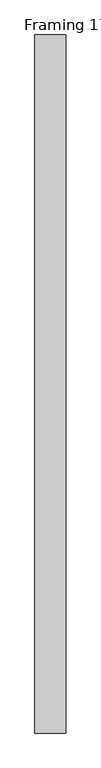
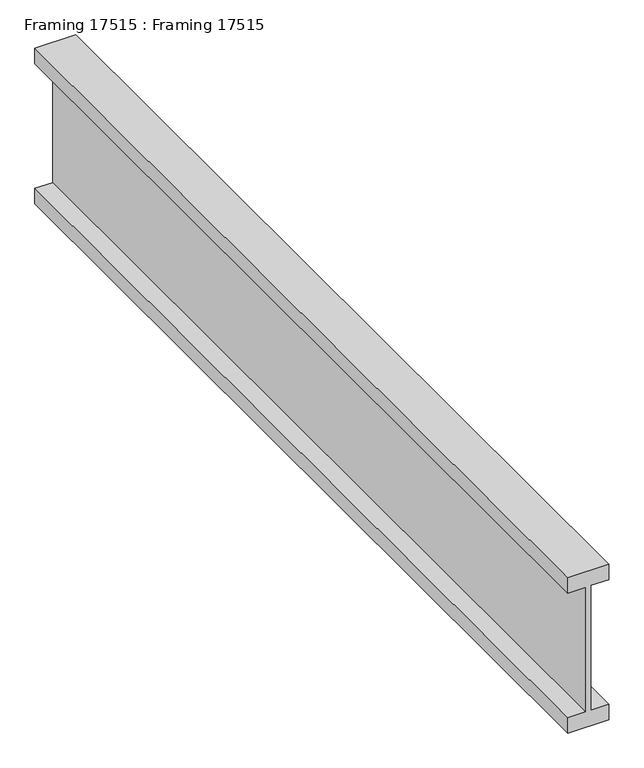
"""IFC4 building model written with IfcOpenShell, lengths in millimetres: proxy geometry, Framing 17515 : Framing 17515."""

from ifc_helpers import new_model, si_unit, frame, origin, place, context, project, spatial, polyline, outline, extrude, source, transform, mapped, element, save


def framing_17515_framing_17515_e96781f7(model_context):
    return source(origin(), model_context, "Body", "SweptSolid", [
        extrude(outline(polyline([(40077.771, 7689.895938), (39792.021, 7689.895938), (39792.021, 7651.002188), (39757.096, 7651.002188), (39757.096, 7739.902188), (39792.021, 7739.902188), (39792.021, 7701.008438), (40077.771, 7701.008438), (40077.771, 7739.902188), (40112.696, 7739.902188), (40112.696, 7651.002188), (40077.771, 7651.002188), (40077.771, 7689.895938)])), frame((0.0, -3747.9491938, 0.0), z_axis=(0.0, 1.0, 0.0), x_axis=(0.0, 0.0, 1.0)), (0.0, 0.0, 1.0), 2000.0),
    ])


if __name__ == "__main__":
    model = new_model("IFC4")
    model_context = context("Model", 3, world=origin())
    ifc_project = project(units=[si_unit("LENGTHUNIT", "METRE", prefix="MILLI")], contexts=[model_context])
    site = spatial("IfcSite", under=ifc_project)
    building = spatial("IfcBuilding", under=site)
    placement = place(None, origin())
    framing_17515_framing_17515_shape = framing_17515_framing_17515_e96781f7(model_context)
    element("IfcBuildingElementProxy", 1, Name="Framing 17515 : Framing 17515", ObjectType="Framing 17515 : Framing 17515", at=placement, inside=building, context=model_context, shape_type="MappedRepresentation", body=[
        mapped(framing_17515_framing_17515_shape, transform((0.0, 0.0, 0.0), x_axis=(1.0, 0.0, 0.0), y_axis=(0.0, 1.0, 0.0), z_axis=(0.0, 0.0, 1.0))),
    ])
    save(model, "model.ifc")

# Revit data of these elements
# Type "Framing 17515 : Framing 17515"
#   NameOverride = "Framing"
# Element 1 (IfcBuildingElementProxy, "Framing 17515 : Framing 17515")
#   Materials on its faces: "WOOD FRAMING (SEE STRUCT DWGS)"
# Materials
#   "WOOD FRAMING (SEE STRUCT DWGS)": class "Unassigned", colour RGB 224 188 168, transparency 0, Cost = 0
